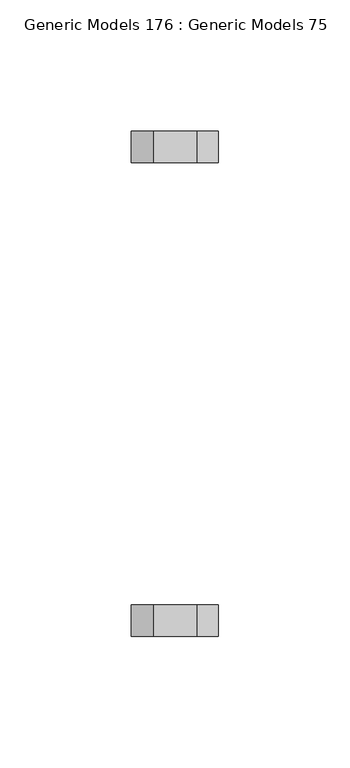
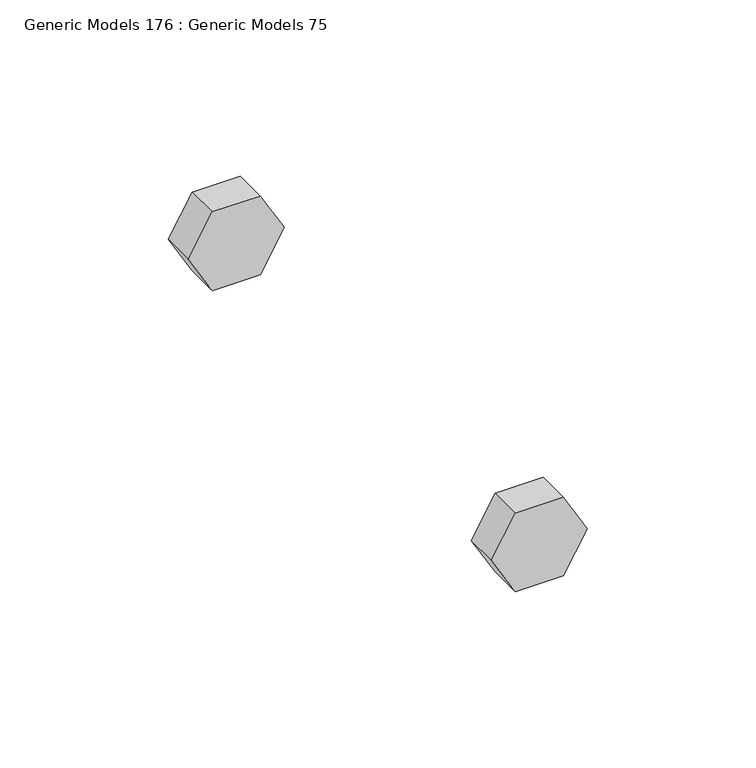
"""IFC4 building model written with IfcOpenShell, lengths in millimetres: proxy geometry, Generic Models 176 : Generic Models 75."""

from ifc_helpers import new_model, si_unit, frame, origin, place, context, project, spatial, polyline, outline, extrude, source, transform, mapped, element, save


def generic_models_176_generic_models_75_eb76e51d(model_context):
    return source(origin(), model_context, "Body", "SweptSolid", [
        extrude(outline(polyline([(271733.9625, 31978.2851858), (271733.9625, 31994.7829698), (271748.25, 32003.0318618), (271762.5375, 31994.7829698), (271762.5375, 31978.2851858), (271748.25, 31970.0362939), (271733.9625, 31978.2851858)])), frame((0.0, 35193.7770442, 0.0), z_axis=(0.0, 1.0, 0.0), x_axis=(0.0, 0.0, 1.0)), (0.0, 0.0, 1.0), 11.90625),
        extrude(outline(polyline([(271733.9625, 31978.2851858), (271733.9625, 31994.7829698), (271748.25, 32003.0318618), (271762.5375, 31994.7829698), (271762.5375, 31978.2851858), (271748.25, 31970.0362939), (271733.9625, 31978.2851858)])), frame((0.0, 35373.9582942, 0.0), z_axis=(0.0, 1.0, 0.0), x_axis=(0.0, 0.0, 1.0)), (0.0, 0.0, 1.0), 11.90625),
    ])


if __name__ == "__main__":
    model = new_model("IFC4")
    model_context = context("Model", 3, world=origin())
    ifc_project = project(units=[si_unit("LENGTHUNIT", "METRE", prefix="MILLI")], contexts=[model_context])
    site = spatial("IfcSite", under=ifc_project)
    building = spatial("IfcBuilding", under=site)
    placement = place(None, origin())
    generic_models_176_generic_models_75_shape = generic_models_176_generic_models_75_eb76e51d(model_context)
    element("IfcBuildingElementProxy", 1, Name="Generic Models 176 : Generic Models 75", ObjectType="Generic Models 176 : Generic Models 75", at=placement, inside=building, context=model_context, shape_type="MappedRepresentation", body=[
        mapped(generic_models_176_generic_models_75_shape, transform((0.0, 0.0, 0.0), x_axis=(1.0, 0.0, 0.0), y_axis=(0.0, 1.0, 0.0), z_axis=(0.0, 0.0, 1.0))),
    ])
    save(model, "model.ifc")

# Revit data of these elements
# Element 1 (IfcBuildingElementProxy, "Generic Models 176 : Generic Models 75")
#   Materials on its faces: "3/4\" GALV. THRU BOLTS"
# Materials
#   "3/4\" GALV. THRU BOLTS": class "Generic", colour RGB 105 69 171, transparency 0, Cost = 0
